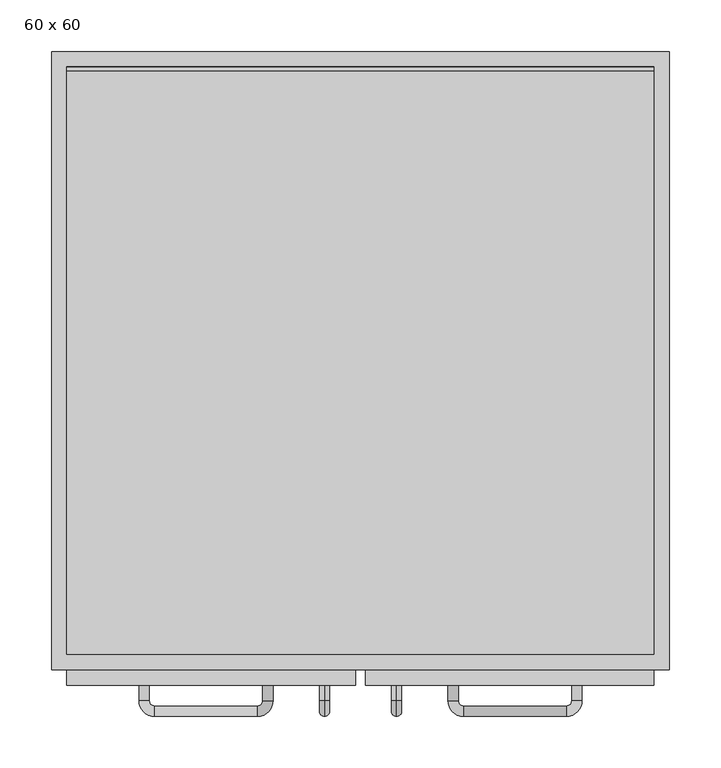
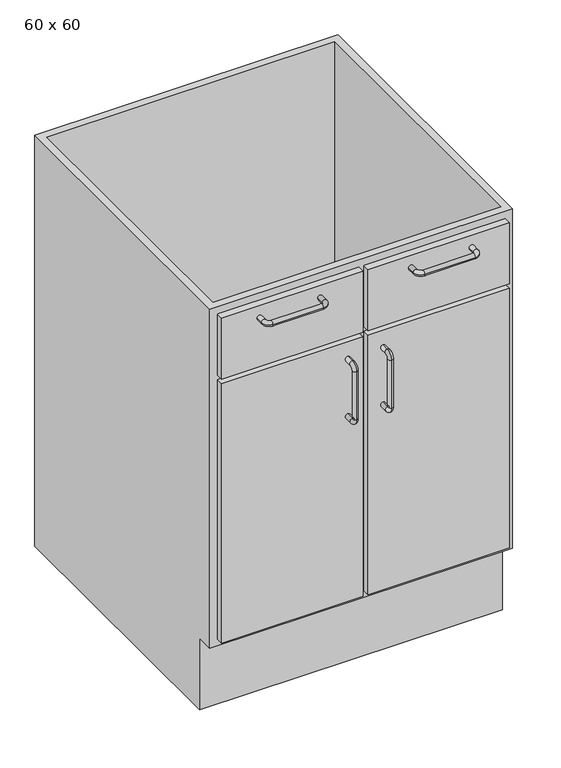
"""IFC4 building model written with IfcOpenShell, lengths in millimetres: furniture geometry, Unterschrank - 2 Schubladen 2 Türen : 60 x 60."""

from ifc_helpers import new_model, si_unit, point, frame, origin, place, context, project, spatial, polyline, circle_curve, ellipse_curve, trimmed, outline, extrude, faceted_brep, source, transform, mapped, element, save
from ifc_brep_helpers import plane_surface, cylinder_surface, revolved_surface, advanced_brep


def furniture_60_x_60_71a814d7(model_context):
    return source(origin(), model_context, "Body", "SolidModel", [
        advanced_brep(
        [(53.7377049, -615.0, 547.5), (53.7377049, -615.0, 557.5), (53.7377049, -630.094, 557.5), (53.7377049, -630.094, 547.5), (53.7377049, -635.0, 562.406), (53.7377049, -645.0, 562.406), (53.7377049, -635.0, 662.594), (53.7377049, -645.0, 662.594), (53.7377049, -630.094, 667.5), (53.7377049, -630.094, 677.5), (53.7377049, -615.0, 677.5), (53.7377049, -615.0, 667.5)],
        [
            (0, 1, circle_curve(frame((53.7377049, -615.0, 552.5), z_axis=(0.0, 1.0, 0.0), x_axis=(0.0, 0.0, 1.0)), 5.0)),
            (1, 0, circle_curve(frame((53.7377049, -615.0, 552.5), z_axis=(0.0, 1.0, 0.0), x_axis=(0.0, 0.0, 1.0)), 5.0)),
            (1, 2),
            (2, 3, circle_curve(frame((53.7377049, -630.094, 552.5), z_axis=(0.0, 1.0, 0.0), x_axis=(0.0, 0.0, 1.0)), 5.0)),
            (3, 0),
            (3, 2, circle_curve(frame((53.7377049, -630.094, 552.5), z_axis=(0.0, 1.0, 0.0), x_axis=(0.0, 0.0, 1.0)), 5.0)),
            (4, 5, circle_curve(frame((53.7377049, -640.0, 562.406), z_axis=(0.0, 0.0, -1.0), x_axis=(0.0, 1.0, 0.0)), 5.0)),
            (5, 3, circle_curve(frame((53.7377049, -630.094, 562.406), z_axis=(1.0, 0.0, 0.0), x_axis=(0.0, 0.0, -1.0)), 14.906)),
            (2, 4, circle_curve(frame((53.7377049, -630.094, 562.406), z_axis=(-1.0, 0.0, 0.0), x_axis=(0.0, 0.0, -1.0)), 4.906)),
            (5, 4, circle_curve(frame((53.7377049, -640.0, 562.406), z_axis=(0.0, 0.0, -1.0), x_axis=(0.0, 1.0, 0.0)), 5.0)),
            (4, 6),
            (6, 7, circle_curve(frame((53.7377049, -640.0, 662.594), z_axis=(0.0, 0.0, -1.0), x_axis=(0.0, 1.0, 0.0)), 5.0)),
            (7, 5),
            (7, 6, circle_curve(frame((53.7377049, -640.0, 662.594), z_axis=(0.0, 0.0, -1.0), x_axis=(0.0, 1.0, 0.0)), 5.0)),
            (8, 9, circle_curve(frame((53.7377049, -630.094, 672.5), z_axis=(0.0, -1.0, 0.0), x_axis=(0.0, 0.0, -1.0)), 5.0)),
            (9, 7, circle_curve(frame((53.7377049, -630.094, 662.594), z_axis=(1.0, 0.0, 0.0), x_axis=(0.0, -1.0, 0.0)), 14.906)),
            (6, 8, circle_curve(frame((53.7377049, -630.094, 662.594), z_axis=(-1.0, 0.0, 0.0), x_axis=(0.0, -1.0, 0.0)), 4.906)),
            (9, 8, circle_curve(frame((53.7377049, -630.094, 672.5), z_axis=(0.0, -1.0, 0.0), x_axis=(0.0, 0.0, -1.0)), 5.0)),
            (10, 11, circle_curve(frame((53.7377049, -615.0, 672.5), z_axis=(0.0, 1.0, 0.0), x_axis=(0.0, 0.0, -1.0)), 5.0)),
            (11, 10, circle_curve(frame((53.7377049, -615.0, 672.5), z_axis=(0.0, 1.0, 0.0), x_axis=(0.0, 0.0, -1.0)), 5.0)),
            (8, 11),
            (10, 9),
        ],
        [
            plane_surface(frame((53.7377049, -615.0, 552.5), z_axis=(0.0, 1.0, 0.0), x_axis=(1.0, 0.0, 0.0))),
            cylinder_surface(frame((53.7377049, -615.0, 552.5), z_axis=(0.0, 1.0, 0.0), x_axis=(0.0, 0.0, 1.0)), 5.0),
            revolved_surface(trimmed(ellipse_curve(frame((53.7377049, -630.094, 552.5), z_axis=(0.0, -1.0, 0.0), x_axis=(0.0, 0.0, 1.0)), 5.0, 5.0), [point((53.7377049, -630.094, 547.5))], [point((53.7377049, -630.094, 557.5))], True, "CARTESIAN"), (53.7377049, -630.094, 562.406), (1.0, 0.0, 0.0)),
            revolved_surface(trimmed(ellipse_curve(frame((53.7377049, -630.094, 552.5), z_axis=(0.0, -1.0, 0.0), x_axis=(0.0, 0.0, 1.0)), 5.0, 5.0), [point((53.7377049, -630.094, 557.5))], [point((53.7377049, -630.094, 547.5))], True, "CARTESIAN"), (53.7377049, -630.094, 562.406), (1.0, 0.0, 0.0)),
            cylinder_surface(frame((53.7377049, -640.0, 562.406), z_axis=(0.0, 0.0, -1.0), x_axis=(0.0, 1.0, 0.0)), 5.0),
            revolved_surface(trimmed(ellipse_curve(frame((53.7377049, -640.0, 662.594), z_axis=(0.0, 0.0, 1.0), x_axis=(0.0, 1.0, 0.0)), 5.0, 5.0), [point((53.7377049, -645.0, 662.594))], [point((53.7377049, -635.0, 662.594))], True, "CARTESIAN"), (53.7377049, -630.094, 662.594), (1.0, 0.0, 0.0)),
            revolved_surface(trimmed(ellipse_curve(frame((53.7377049, -640.0, 662.594), z_axis=(0.0, 0.0, 1.0), x_axis=(0.0, 1.0, 0.0)), 5.0, 5.0), [point((53.7377049, -635.0, 662.594))], [point((53.7377049, -645.0, 662.594))], True, "CARTESIAN"), (53.7377049, -630.094, 662.594), (1.0, 0.0, 0.0)),
            plane_surface(frame((53.7377049, -615.0, 672.5), z_axis=(0.0, 1.0, 0.0), x_axis=(1.0, 0.0, 0.0))),
            cylinder_surface(frame((53.7377049, -630.094, 672.5), z_axis=(0.0, -1.0, 0.0), x_axis=(0.0, 0.0, -1.0)), 5.0),
        ],
        [
            (0, [[1, 2]]),
            (1, [[3, 4, 5, -2]]),
            (1, [[-5, 6, -3, -1]]),
            (2, [[7, 8, -4, 9]]),
            (3, [[10, -9, -6, -8]]),
            (4, [[11, 12, 13, -7]]),
            (4, [[-13, 14, -11, -10]]),
            (5, [[15, 16, -12, 17]]),
            (6, [[18, -17, -14, -16]]),
            (7, [[19, 20]]),
            (8, [[21, -19, 22, -15]]),
            (8, [[-22, -20, -21, -18]]),
        ],
    ),
        advanced_brep(
        [(103.7377049, -615.0, 820.0), (113.7377049, -615.0, 820.0), (113.7377049, -630.094, 820.0), (103.7377049, -630.094, 820.0), (118.6437049, -635.0, 820.0), (118.6437049, -645.0, 820.0), (218.8317049, -635.0, 820.0), (218.8317049, -645.0, 820.0), (223.7377049, -630.094, 820.0), (233.7377049, -630.094, 820.0), (233.7377049, -615.0, 820.0), (223.7377049, -615.0, 820.0)],
        [
            (0, 1, circle_curve(frame((108.7377049, -615.0, 820.0), z_axis=(0.0, 1.0, 0.0), x_axis=(1.0, 0.0, 0.0)), 5.0)),
            (1, 0, circle_curve(frame((108.7377049, -615.0, 820.0), z_axis=(0.0, 1.0, 0.0), x_axis=(1.0, 0.0, 0.0)), 5.0)),
            (1, 2),
            (2, 3, circle_curve(frame((108.7377049, -630.094, 820.0), z_axis=(0.0, 1.0, 0.0), x_axis=(1.0, 0.0, 0.0)), 5.0)),
            (3, 0),
            (3, 2, circle_curve(frame((108.7377049, -630.094, 820.0), z_axis=(0.0, 1.0, 0.0), x_axis=(1.0, 0.0, 0.0)), 5.0)),
            (4, 5, circle_curve(frame((118.6437049, -640.0, 820.0), z_axis=(-1.0, 0.0, 0.0), x_axis=(0.0, 1.0, 0.0)), 5.0)),
            (5, 3, circle_curve(frame((118.6437049, -630.094, 820.0), z_axis=(0.0, 0.0, -1.0), x_axis=(-1.0, 0.0, 0.0)), 14.906)),
            (2, 4, circle_curve(frame((118.6437049, -630.094, 820.0), z_axis=(0.0, 0.0, 1.0), x_axis=(-1.0, 0.0, 0.0)), 4.906)),
            (5, 4, circle_curve(frame((118.6437049, -640.0, 820.0), z_axis=(-1.0, 0.0, 0.0), x_axis=(0.0, 1.0, 0.0)), 5.0)),
            (4, 6),
            (6, 7, circle_curve(frame((218.8317049, -640.0, 820.0), z_axis=(-1.0, 0.0, 0.0), x_axis=(0.0, 1.0, 0.0)), 5.0)),
            (7, 5),
            (7, 6, circle_curve(frame((218.8317049, -640.0, 820.0), z_axis=(-1.0, 0.0, 0.0), x_axis=(0.0, 1.0, 0.0)), 5.0)),
            (8, 9, circle_curve(frame((228.7377049, -630.094, 820.0), z_axis=(0.0, -1.0, 0.0), x_axis=(-1.0, 0.0, 0.0)), 5.0)),
            (9, 7, circle_curve(frame((218.8317049, -630.094, 820.0), z_axis=(0.0, 0.0, -1.0), x_axis=(0.0, -1.0, 0.0)), 14.906)),
            (6, 8, circle_curve(frame((218.8317049, -630.094, 820.0), z_axis=(0.0, 0.0, 1.0), x_axis=(0.0, -1.0, 0.0)), 4.906)),
            (9, 8, circle_curve(frame((228.7377049, -630.094, 820.0), z_axis=(0.0, -1.0, 0.0), x_axis=(-1.0, 0.0, 0.0)), 5.0)),
            (10, 11, circle_curve(frame((228.7377049, -615.0, 820.0), z_axis=(0.0, 1.0, 0.0), x_axis=(-1.0, 0.0, 0.0)), 5.0)),
            (11, 10, circle_curve(frame((228.7377049, -615.0, 820.0), z_axis=(0.0, 1.0, 0.0), x_axis=(-1.0, 0.0, 0.0)), 5.0)),
            (8, 11),
            (10, 9),
        ],
        [
            plane_surface(frame((108.7377049, -615.0, 820.0), z_axis=(0.0, 1.0, 0.0), x_axis=(0.0, 0.0, 1.0))),
            cylinder_surface(frame((108.7377049, -615.0, 820.0), z_axis=(0.0, 1.0, 0.0), x_axis=(1.0, 0.0, 0.0)), 5.0),
            revolved_surface(trimmed(ellipse_curve(frame((108.7377049, -630.094, 820.0), z_axis=(0.0, -1.0, 0.0), x_axis=(1.0, 0.0, 0.0)), 5.0, 5.0), [point((103.7377049, -630.094, 820.0))], [point((113.7377049, -630.094, 820.0))], True, "CARTESIAN"), (118.6437049, -630.094, 820.0), (0.0, 0.0, -1.0)),
            revolved_surface(trimmed(ellipse_curve(frame((108.7377049, -630.094, 820.0), z_axis=(0.0, -1.0, 0.0), x_axis=(1.0, 0.0, 0.0)), 5.0, 5.0), [point((113.7377049, -630.094, 820.0))], [point((103.7377049, -630.094, 820.0))], True, "CARTESIAN"), (118.6437049, -630.094, 820.0), (0.0, 0.0, -1.0)),
            cylinder_surface(frame((118.6437049, -640.0, 820.0), z_axis=(-1.0, 0.0, 0.0), x_axis=(0.0, 1.0, 0.0)), 5.0),
            revolved_surface(trimmed(ellipse_curve(frame((218.8317049, -640.0, 820.0), z_axis=(1.0, 0.0, 0.0), x_axis=(0.0, 1.0, 0.0)), 5.0, 5.0), [point((218.8317049, -645.0, 820.0))], [point((218.8317049, -635.0, 820.0))], True, "CARTESIAN"), (218.8317049, -630.094, 820.0), (0.0, 0.0, -1.0)),
            revolved_surface(trimmed(ellipse_curve(frame((218.8317049, -640.0, 820.0), z_axis=(1.0, 0.0, 0.0), x_axis=(0.0, 1.0, 0.0)), 5.0, 5.0), [point((218.8317049, -635.0, 820.0))], [point((218.8317049, -645.0, 820.0))], True, "CARTESIAN"), (218.8317049, -630.094, 820.0), (0.0, 0.0, -1.0)),
            plane_surface(frame((228.7377049, -615.0, 820.0), z_axis=(0.0, 1.0, 0.0), x_axis=(0.0, 0.0, 1.0))),
            cylinder_surface(frame((228.7377049, -630.094, 820.0), z_axis=(0.0, -1.0, 0.0), x_axis=(-1.0, 0.0, 0.0)), 5.0),
        ],
        [
            (0, [[1, 2]]),
            (1, [[3, 4, 5, -2]]),
            (1, [[-5, 6, -3, -1]]),
            (2, [[7, 8, -4, 9]]),
            (3, [[10, -9, -6, -8]]),
            (4, [[11, 12, 13, -7]]),
            (4, [[-13, 14, -11, -10]]),
            (5, [[15, 16, -12, 17]]),
            (6, [[18, -17, -14, -16]]),
            (7, [[19, 20]]),
            (8, [[21, -19, 22, -15]]),
            (8, [[-22, -20, -21, -18]]),
        ],
    ),
        advanced_brep(
        [(-66.2622951, -615.0, 820.0), (-76.2622951, -615.0, 820.0), (-66.2622951, -630.094, 820.0), (-76.2622951, -630.094, 820.0), (-81.1682951, -635.0, 820.0), (-81.1682951, -645.0, 820.0), (-181.3562951, -645.0, 820.0), (-181.3562951, -635.0, 820.0), (-186.2622951, -630.094, 820.0), (-196.2622951, -630.094, 820.0), (-196.2622951, -615.0, 820.0), (-186.2622951, -615.0, 820.0)],
        [
            (0, 1, circle_curve(frame((-71.2622951, -615.0, 820.0), z_axis=(0.0, 1.0, 0.0), x_axis=(-1.0, 0.0, 0.0)), 5.0)),
            (1, 0, circle_curve(frame((-71.2622951, -615.0, 820.0), z_axis=(0.0, 1.0, 0.0), x_axis=(-1.0, 0.0, 0.0)), 5.0)),
            (0, 2),
            (2, 3, circle_curve(frame((-71.2622951, -630.094, 820.0), z_axis=(0.0, 1.0, 0.0), x_axis=(-1.0, 0.0, 0.0)), 5.0)),
            (3, 1),
            (3, 2, circle_curve(frame((-71.2622951, -630.094, 820.0), z_axis=(0.0, 1.0, 0.0), x_axis=(-1.0, 0.0, 0.0)), 5.0)),
            (4, 3, circle_curve(frame((-81.1682951, -630.094, 820.0), z_axis=(0.0, 0.0, 1.0), x_axis=(1.0, 0.0, 0.0)), 4.906)),
            (2, 5, circle_curve(frame((-81.1682951, -630.094, 820.0), z_axis=(0.0, 0.0, -1.0), x_axis=(1.0, 0.0, 0.0)), 14.906)),
            (5, 4, circle_curve(frame((-81.1682951, -640.0, 820.0), z_axis=(1.0, 0.0, 0.0), x_axis=(0.0, 1.0, 0.0)), 5.0)),
            (4, 5, circle_curve(frame((-81.1682951, -640.0, 820.0), z_axis=(1.0, 0.0, 0.0), x_axis=(0.0, 1.0, 0.0)), 5.0)),
            (5, 6),
            (6, 7, circle_curve(frame((-181.3562951, -640.0, 820.0), z_axis=(1.0, 0.0, 0.0), x_axis=(0.0, 1.0, 0.0)), 5.0)),
            (7, 4),
            (7, 6, circle_curve(frame((-181.3562951, -640.0, 820.0), z_axis=(1.0, 0.0, 0.0), x_axis=(0.0, 1.0, 0.0)), 5.0)),
            (8, 7, circle_curve(frame((-181.3562951, -630.094, 820.0), z_axis=(0.0, 0.0, 1.0), x_axis=(0.0, -1.0, 0.0)), 4.906)),
            (6, 9, circle_curve(frame((-181.3562951, -630.094, 820.0), z_axis=(0.0, 0.0, -1.0), x_axis=(0.0, -1.0, 0.0)), 14.906)),
            (9, 8, circle_curve(frame((-191.2622951, -630.094, 820.0), z_axis=(0.0, -1.0, 0.0), x_axis=(1.0, 0.0, 0.0)), 5.0)),
            (8, 9, circle_curve(frame((-191.2622951, -630.094, 820.0), z_axis=(0.0, -1.0, 0.0), x_axis=(1.0, 0.0, 0.0)), 5.0)),
            (10, 11, circle_curve(frame((-191.2622951, -615.0, 820.0), z_axis=(0.0, 1.0, 0.0), x_axis=(1.0, 0.0, 0.0)), 5.0)),
            (11, 10, circle_curve(frame((-191.2622951, -615.0, 820.0), z_axis=(0.0, 1.0, 0.0), x_axis=(1.0, 0.0, 0.0)), 5.0)),
            (9, 10),
            (11, 8),
        ],
        [
            plane_surface(frame((-71.2622951, -615.0, 820.0), z_axis=(0.0, 1.0, 0.0), x_axis=(0.0, 0.0, 1.0))),
            cylinder_surface(frame((-71.2622951, -615.0, 820.0), z_axis=(0.0, 1.0, 0.0), x_axis=(-1.0, 0.0, 0.0)), 5.0),
            revolved_surface(trimmed(ellipse_curve(frame((-71.2622951, -630.094, 820.0), z_axis=(0.0, 1.0, 0.0), x_axis=(-1.0, 0.0, 0.0)), 5.0, 5.0), [point((-66.2622951, -630.094, 820.0))], [point((-76.2622951, -630.094, 820.0))], True, "CARTESIAN"), (-81.1682951, -630.094, 820.0), (0.0, 0.0, -1.0)),
            revolved_surface(trimmed(ellipse_curve(frame((-71.2622951, -630.094, 820.0), z_axis=(0.0, 1.0, 0.0), x_axis=(-1.0, 0.0, 0.0)), 5.0, 5.0), [point((-76.2622951, -630.094, 820.0))], [point((-66.2622951, -630.094, 820.0))], True, "CARTESIAN"), (-81.1682951, -630.094, 820.0), (0.0, 0.0, -1.0)),
            cylinder_surface(frame((-81.1682951, -640.0, 820.0), z_axis=(1.0, 0.0, 0.0), x_axis=(0.0, 1.0, 0.0)), 5.0),
            revolved_surface(trimmed(ellipse_curve(frame((-181.3562951, -640.0, 820.0), z_axis=(1.0, 0.0, 0.0), x_axis=(0.0, 1.0, 0.0)), 5.0, 5.0), [point((-181.3562951, -645.0, 820.0))], [point((-181.3562951, -635.0, 820.0))], True, "CARTESIAN"), (-181.3562951, -630.094, 820.0), (0.0, 0.0, -1.0)),
            revolved_surface(trimmed(ellipse_curve(frame((-181.3562951, -640.0, 820.0), z_axis=(1.0, 0.0, 0.0), x_axis=(0.0, 1.0, 0.0)), 5.0, 5.0), [point((-181.3562951, -635.0, 820.0))], [point((-181.3562951, -645.0, 820.0))], True, "CARTESIAN"), (-181.3562951, -630.094, 820.0), (0.0, 0.0, -1.0)),
            plane_surface(frame((-191.2622951, -615.0, 820.0), z_axis=(0.0, 1.0, 0.0), x_axis=(0.0, 0.0, 1.0))),
            cylinder_surface(frame((-191.2622951, -630.094, 820.0), z_axis=(0.0, -1.0, 0.0), x_axis=(1.0, 0.0, 0.0)), 5.0),
        ],
        [
            (0, [[1, 2]]),
            (1, [[-1, 3, 4, 5]]),
            (1, [[-2, -5, 6, -3]]),
            (2, [[7, -4, 8, 9]]),
            (3, [[-8, -6, -7, 10]]),
            (4, [[-9, 11, 12, 13]]),
            (4, [[-10, -13, 14, -11]]),
            (5, [[15, -12, 16, 17]]),
            (6, [[-16, -14, -15, 18]]),
            (7, [[19, 20]]),
            (8, [[-17, 21, -20, 22]]),
            (8, [[-18, -22, -19, -21]]),
        ],
    ),
        advanced_brep(
        [(-16.2622951, -615.0, 547.5), (-16.2622951, -615.0, 557.5), (-16.2622951, -630.094, 547.5), (-16.2622951, -630.094, 557.5), (-16.2622951, -635.0, 562.406), (-16.2622951, -645.0, 562.406), (-16.2622951, -645.0, 662.594), (-16.2622951, -635.0, 662.594), (-16.2622951, -630.094, 667.5), (-16.2622951, -630.094, 677.5), (-16.2622951, -615.0, 677.5), (-16.2622951, -615.0, 667.5)],
        [
            (0, 1, circle_curve(frame((-16.2622951, -615.0, 552.5), z_axis=(0.0, 1.0, 0.0), x_axis=(0.0, 0.0, 1.0)), 5.0)),
            (1, 0, circle_curve(frame((-16.2622951, -615.0, 552.5), z_axis=(0.0, 1.0, 0.0), x_axis=(0.0, 0.0, 1.0)), 5.0)),
            (0, 2),
            (2, 3, circle_curve(frame((-16.2622951, -630.094, 552.5), z_axis=(0.0, 1.0, 0.0), x_axis=(0.0, 0.0, 1.0)), 5.0)),
            (3, 1),
            (3, 2, circle_curve(frame((-16.2622951, -630.094, 552.5), z_axis=(0.0, 1.0, 0.0), x_axis=(0.0, 0.0, 1.0)), 5.0)),
            (4, 3, circle_curve(frame((-16.2622951, -630.094, 562.406), z_axis=(1.0, 0.0, 0.0), x_axis=(0.0, 0.0, -1.0)), 4.906)),
            (2, 5, circle_curve(frame((-16.2622951, -630.094, 562.406), z_axis=(-1.0, 0.0, 0.0), x_axis=(0.0, 0.0, -1.0)), 14.906)),
            (5, 4, circle_curve(frame((-16.2622951, -640.0, 562.406), z_axis=(0.0, 0.0, -1.0), x_axis=(0.0, 1.0, 0.0)), 5.0)),
            (4, 5, circle_curve(frame((-16.2622951, -640.0, 562.406), z_axis=(0.0, 0.0, -1.0), x_axis=(0.0, 1.0, 0.0)), 5.0)),
            (5, 6),
            (6, 7, circle_curve(frame((-16.2622951, -640.0, 662.594), z_axis=(0.0, 0.0, -1.0), x_axis=(0.0, 1.0, 0.0)), 5.0)),
            (7, 4),
            (7, 6, circle_curve(frame((-16.2622951, -640.0, 662.594), z_axis=(0.0, 0.0, -1.0), x_axis=(0.0, 1.0, 0.0)), 5.0)),
            (8, 7, circle_curve(frame((-16.2622951, -630.094, 662.594), z_axis=(1.0, 0.0, 0.0), x_axis=(0.0, -1.0, 0.0)), 4.906)),
            (6, 9, circle_curve(frame((-16.2622951, -630.094, 662.594), z_axis=(-1.0, 0.0, 0.0), x_axis=(0.0, -1.0, 0.0)), 14.906)),
            (9, 8, circle_curve(frame((-16.2622951, -630.094, 672.5), z_axis=(0.0, -1.0, 0.0), x_axis=(0.0, 0.0, -1.0)), 5.0)),
            (8, 9, circle_curve(frame((-16.2622951, -630.094, 672.5), z_axis=(0.0, -1.0, 0.0), x_axis=(0.0, 0.0, -1.0)), 5.0)),
            (10, 11, circle_curve(frame((-16.2622951, -615.0, 672.5), z_axis=(0.0, 1.0, 0.0), x_axis=(0.0, 0.0, -1.0)), 5.0)),
            (11, 10, circle_curve(frame((-16.2622951, -615.0, 672.5), z_axis=(0.0, 1.0, 0.0), x_axis=(0.0, 0.0, -1.0)), 5.0)),
            (9, 10),
            (11, 8),
        ],
        [
            plane_surface(frame((-16.2622951, -615.0, 552.5), z_axis=(0.0, 1.0, 0.0), x_axis=(-1.0, 0.0, 0.0))),
            cylinder_surface(frame((-16.2622951, -615.0, 552.5), z_axis=(0.0, 1.0, 0.0), x_axis=(0.0, 0.0, 1.0)), 5.0),
            revolved_surface(trimmed(ellipse_curve(frame((-16.2622951, -630.094, 552.5), z_axis=(0.0, 1.0, 0.0), x_axis=(0.0, 0.0, 1.0)), 5.0, 5.0), [point((-16.2622951, -630.094, 547.5))], [point((-16.2622951, -630.094, 557.5))], True, "CARTESIAN"), (-16.2622951, -630.094, 562.406), (-1.0, 0.0, 0.0)),
            revolved_surface(trimmed(ellipse_curve(frame((-16.2622951, -630.094, 552.5), z_axis=(0.0, 1.0, 0.0), x_axis=(0.0, 0.0, 1.0)), 5.0, 5.0), [point((-16.2622951, -630.094, 557.5))], [point((-16.2622951, -630.094, 547.5))], True, "CARTESIAN"), (-16.2622951, -630.094, 562.406), (-1.0, 0.0, 0.0)),
            cylinder_surface(frame((-16.2622951, -640.0, 562.406), z_axis=(0.0, 0.0, -1.0), x_axis=(0.0, 1.0, 0.0)), 5.0),
            revolved_surface(trimmed(ellipse_curve(frame((-16.2622951, -640.0, 662.594), z_axis=(0.0, 0.0, -1.0), x_axis=(0.0, 1.0, 0.0)), 5.0, 5.0), [point((-16.2622951, -645.0, 662.594))], [point((-16.2622951, -635.0, 662.594))], True, "CARTESIAN"), (-16.2622951, -630.094, 662.594), (-1.0, 0.0, 0.0)),
            revolved_surface(trimmed(ellipse_curve(frame((-16.2622951, -640.0, 662.594), z_axis=(0.0, 0.0, -1.0), x_axis=(0.0, 1.0, 0.0)), 5.0, 5.0), [point((-16.2622951, -635.0, 662.594))], [point((-16.2622951, -645.0, 662.594))], True, "CARTESIAN"), (-16.2622951, -630.094, 662.594), (-1.0, 0.0, 0.0)),
            plane_surface(frame((-16.2622951, -615.0, 672.5), z_axis=(0.0, 1.0, 0.0), x_axis=(-1.0, 0.0, 0.0))),
            cylinder_surface(frame((-16.2622951, -630.094, 672.5), z_axis=(0.0, -1.0, 0.0), x_axis=(0.0, 0.0, -1.0)), 5.0),
        ],
        [
            (0, [[1, 2]]),
            (1, [[-1, 3, 4, 5]]),
            (1, [[-2, -5, 6, -3]]),
            (2, [[7, -4, 8, 9]]),
            (3, [[-8, -6, -7, 10]]),
            (4, [[-9, 11, 12, 13]]),
            (4, [[-10, -13, 14, -11]]),
            (5, [[15, -12, 16, 17]]),
            (6, [[-16, -14, -15, 18]]),
            (7, [[19, 20]]),
            (8, [[-17, 21, -20, 22]]),
            (8, [[-18, -22, -19, -21]]),
        ],
    ),
        faceted_brep([(303.7377049, -19.05, 165.0), (-266.2622951, -19.05, 165.0), (-266.2622951, -585.0, 165.0), (303.7377049, -585.0, 165.0), (318.7377049, -600.0, 150.0), (-281.2622951, -600.0, 150.0), (-281.2622951, -565.0, 150.0), (318.7377049, -565.0, 150.0), (303.7377049, -19.05, 150.0), (-266.2622951, -19.05, 150.0), (318.7377049, -600.0, 860.0), (318.7377049, 0.0, 860.0), (-281.2622951, 0.0, 860.0), (-281.2622951, -600.0, 860.0), (-266.2622951, -15.0, 860.0), (303.7377049, -15.0, 860.0), (303.7377049, -585.0, 860.0), (-266.2622951, -585.0, 860.0), (-266.2622951, -15.0, 150.0), (303.7377049, -15.0, 150.0), (318.7377049, -565.0, 0.0), (318.7377049, 0.0, 0.0), (-281.2622951, 0.0, 0.0), (-281.2622951, -565.0, 0.0)], [[[0, 1, 2, 3]], [[4, 5, 6, 7]], [[1, 0, 8, 9]], [[10, 11, 12, 13], [14, 15, 16, 17]], [[14, 17, 2, 1, 9, 18]], [[15, 14, 18, 19]], [[16, 15, 19, 8, 0, 3]], [[11, 10, 4, 7, 20, 21]], [[12, 11, 21, 22]], [[13, 12, 22, 23, 6, 5]], [[10, 13, 5, 4]], [[17, 16, 3, 2]], [[9, 8, 19, 18]], [[21, 20, 23, 22]], [[23, 20, 7, 6]]]),
        extrude(outline(polyline([(13.7377049, -615.0), (-266.2622951, -615.0), (-266.2622951, -600.0), (13.7377049, -600.0), (13.7377049, -615.0)])), frame((0.0, 0.0, 717.5), z_axis=(0.0, 0.0, 1.0), x_axis=(1.0, 0.0, 0.0)), (0.0, 0.0, 1.0), 127.5),
        extrude(outline(polyline([(303.7377049, -615.0), (23.7377049, -615.0), (23.7377049, -600.0), (303.7377049, -600.0), (303.7377049, -615.0)])), frame((0.0, 0.0, 717.5), z_axis=(0.0, 0.0, 1.0), x_axis=(1.0, 0.0, 0.0)), (0.0, 0.0, 1.0), 127.5),
        extrude(outline(polyline([(13.7377049, -615.0), (-266.2622951, -615.0), (-266.2622951, -600.0), (13.7377049, -600.0), (13.7377049, -615.0)])), frame((0.0, 0.0, 165.0), z_axis=(0.0, 0.0, 1.0), x_axis=(1.0, 0.0, 0.0)), (0.0, 0.0, 1.0), 542.5),
        extrude(outline(polyline([(303.7377049, -615.0), (23.7377049, -615.0), (23.7377049, -600.0), (303.7377049, -600.0), (303.7377049, -615.0)])), frame((0.0, 0.0, 165.0), z_axis=(0.0, 0.0, 1.0), x_axis=(1.0, 0.0, 0.0)), (0.0, 0.0, 1.0), 542.5),
    ])


if __name__ == "__main__":
    model = new_model("IFC4")
    model_context = context("Model", 3, world=origin())
    ifc_project = project(units=[si_unit("LENGTHUNIT", "METRE", prefix="MILLI")], contexts=[model_context])
    site = spatial("IfcSite", under=ifc_project)
    building = spatial("IfcBuilding", under=site)
    placement = place(None, origin())
    furniture_60_x_60_shape = furniture_60_x_60_71a814d7(model_context)
    element("IfcFurniture", 1, ObjectType="Unterschrank - 2 Schubladen 2 Türen : 60 x 60", at=placement, inside=building, context=model_context, shape_type="MappedRepresentation", body=[
        mapped(furniture_60_x_60_shape, transform((0.0, 0.0, 0.0), x_axis=(1.0, 0.0, 0.0), y_axis=(0.0, 1.0, 0.0), z_axis=(0.0, 0.0, 1.0))),
    ])
    save(model, "model.ifc")

# Revit data of these elements
# Type "Unterschrank - 2 Schubladen 2 Türen : 60 x 60"
#   Depth = 0.600 m
#   Height = 0.860 m
#   Sockeltiefe = 0.035 m
#   Sockelhöhe = 0.150 m
#   Width = 0.600 m
#   Corpus = Kunststoff - Glatt - Weiß
#   Vorn = Kunststoff - Glatt - Weiß
#   Griff = Metall - Aluminium
# Element 1 (IfcFurniture, "Unterschrank - 2 Schubladen 2 Türen : 60 x 60")
#   Materials on its faces: "Metall - Aluminium", "Kunststoff - Glatt - Weiß"
# Materials
#   "Kunststoff - Glatt - Weiß": class "Metall", colour RGB 234 234 234, transparency 0
#   "Metall - Aluminium": class "Metall", colour RGB 247 247 247, transparency 0, Description = "Aluminium 6061", Cost = 0
